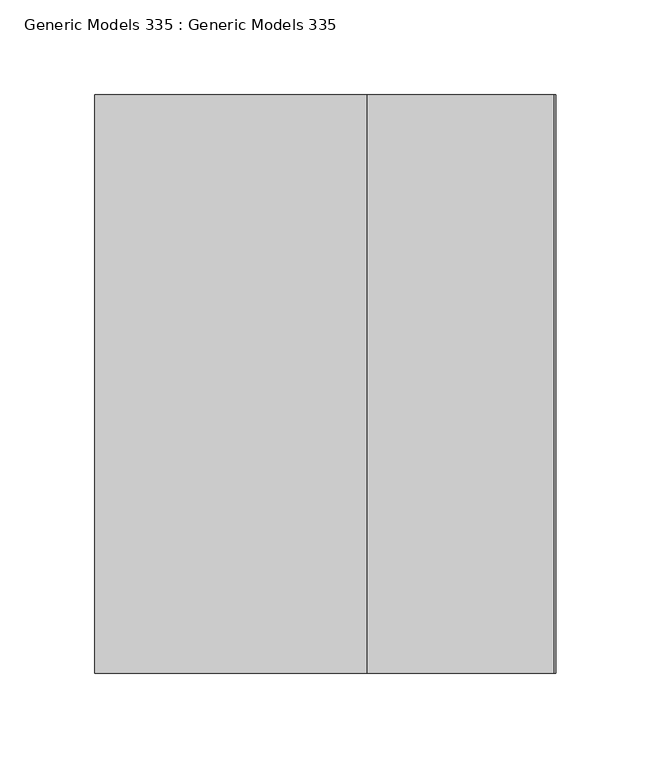
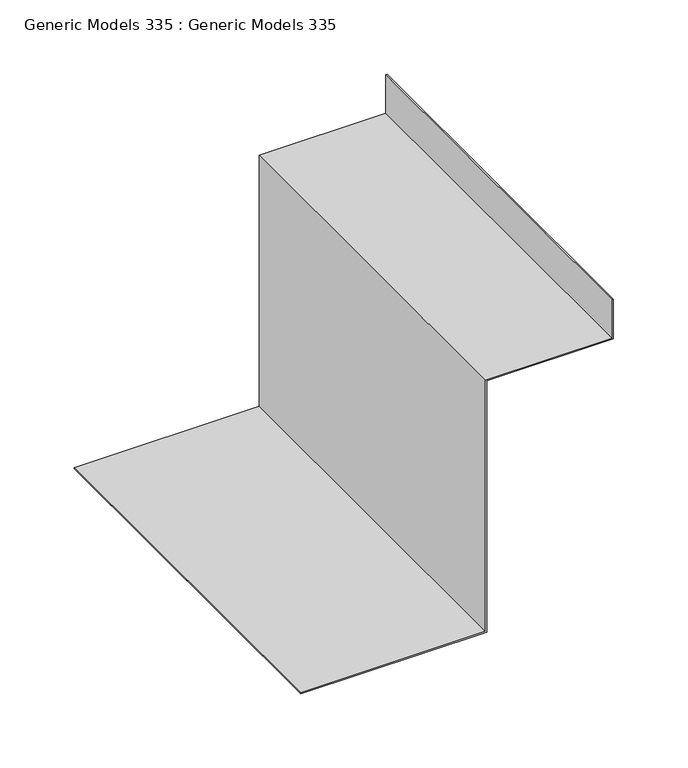
"""IFC4 building model written with IfcOpenShell, lengths in millimetres: proxy geometry, Generic Models 335 : Generic Models 335."""

from ifc_helpers import new_model, si_unit, frame, origin, place, context, project, spatial, polyline, outline, extrude, source, transform, mapped, element, save


def generic_models_335_generic_models_335_61fdec5c(model_context):
    return source(origin(), model_context, "Body", "SweptSolid", [
        extrude(outline(polyline([(126362.9890926, 8573.99027), (126362.9890926, 8475.3803327), (126156.5985119, 8475.3803327), (126156.5985119, 8331.7518122), (126155.6850616, 8331.7518122), (126155.6850616, 8476.3057313), (126362.2084204, 8476.3057313), (126362.2084204, 8574.8314203), (126394.7390926, 8574.8314203), (126394.7390926, 8573.99027), (126362.9890926, 8573.99027)])), frame((0.0, -4109.6428838, 0.0), z_axis=(0.0, 1.0, 0.0), x_axis=(0.0, 0.0, 1.0)), (0.0, 0.0, 1.0), 304.8),
    ])


if __name__ == "__main__":
    model = new_model("IFC4")
    model_context = context("Model", 3, world=origin())
    ifc_project = project(units=[si_unit("LENGTHUNIT", "METRE", prefix="MILLI")], contexts=[model_context])
    site = spatial("IfcSite", under=ifc_project)
    building = spatial("IfcBuilding", under=site)
    placement = place(None, origin())
    generic_models_335_generic_models_335_shape = generic_models_335_generic_models_335_61fdec5c(model_context)
    element("IfcBuildingElementProxy", 1, Name="Generic Models 335 : Generic Models 335", ObjectType="Generic Models 335 : Generic Models 335", at=placement, inside=building, context=model_context, shape_type="MappedRepresentation", body=[
        mapped(generic_models_335_generic_models_335_shape, transform((0.0, 0.0, 0.0), x_axis=(1.0, 0.0, 0.0), y_axis=(0.0, 1.0, 0.0), z_axis=(0.0, 0.0, 1.0))),
    ])
    save(model, "model.ifc")

# Revit data of these elements
# Element 1 (IfcBuildingElementProxy, "Generic Models 335 : Generic Models 335")
#   Materials on its faces: "_(2) LAYERS NO. 30 ASTM D226 ASPHALT SATURATED ORGANIC FELT"
# Materials
#   "_(2) LAYERS NO. 30 ASTM D226 ASPHALT SATURATED ORGANIC FELT": class "Generic", colour RGB 67 154 161, transparency 0, Cost = 0
